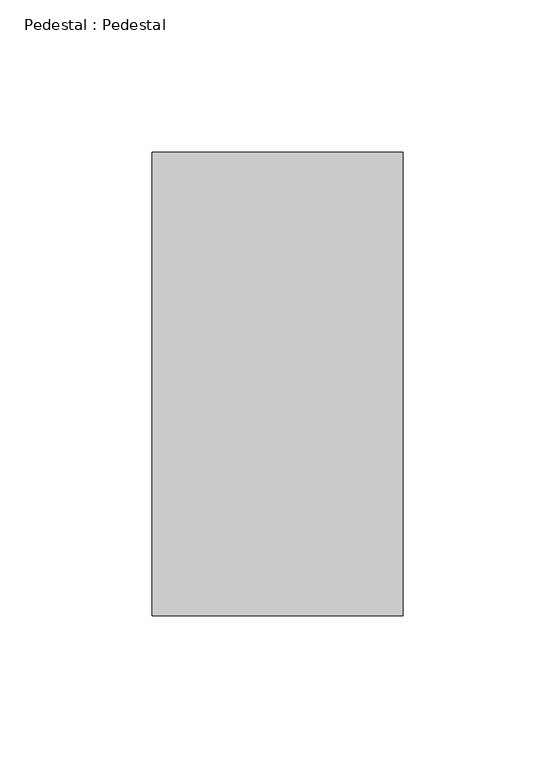
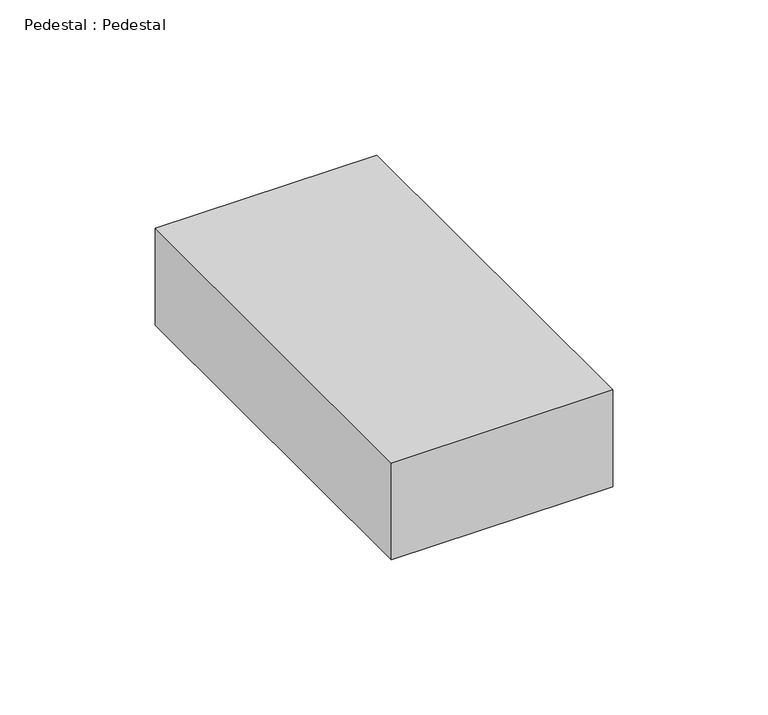
"""IFC4 building model written with IfcOpenShell, lengths in millimetres: proxy geometry, Pedestal : Pedestal."""

from ifc_helpers import new_model, si_unit, frame, origin, place, context, project, spatial, polyline, outline, extrude, source, transform, mapped, element, save


def pedestal_pedestal_c426ac54(model_context):
    return source(origin(), model_context, "Body", "SweptSolid", [
        extrude(outline(polyline([(-9662.4978516, 9829.7531721), (-9745.0478516, 9829.7531721), (-9745.0478516, 9982.1531721), (-9662.4978516, 9982.1531721), (-9662.4978516, 9829.7531721)])), frame((0.0, 0.0, 40107.9492187), z_axis=(0.0, 0.0, 1.0), x_axis=(1.0, 0.0, 0.0)), (0.0, 0.0, 1.0), 38.1),
    ])


if __name__ == "__main__":
    model = new_model("IFC4")
    model_context = context("Model", 3, world=origin())
    ifc_project = project(units=[si_unit("LENGTHUNIT", "METRE", prefix="MILLI")], contexts=[model_context])
    site = spatial("IfcSite", under=ifc_project)
    building = spatial("IfcBuilding", under=site)
    placement = place(None, origin())
    pedestal_pedestal_shape = pedestal_pedestal_c426ac54(model_context)
    element("IfcBuildingElementProxy", 1, Name="Pedestal : Pedestal", ObjectType="Pedestal : Pedestal", at=placement, inside=building, context=model_context, shape_type="MappedRepresentation", body=[
        mapped(pedestal_pedestal_shape, transform((0.0, 0.0, 0.0), x_axis=(1.0, 0.0, 0.0), y_axis=(0.0, 1.0, 0.0), z_axis=(0.0, 0.0, 1.0))),
    ])
    save(model, "model.ifc")

# Revit data of these elements
# Type "Pedestal : Pedestal"
#   NameOverride = "Pedestal"
# Element 1 (IfcBuildingElementProxy, "Pedestal : Pedestal")
#   Materials on its faces: "BUZON PEDESTAL"
# Materials
#   "BUZON PEDESTAL": class "Unassigned", colour RGB 66 66 66, transparency 0
